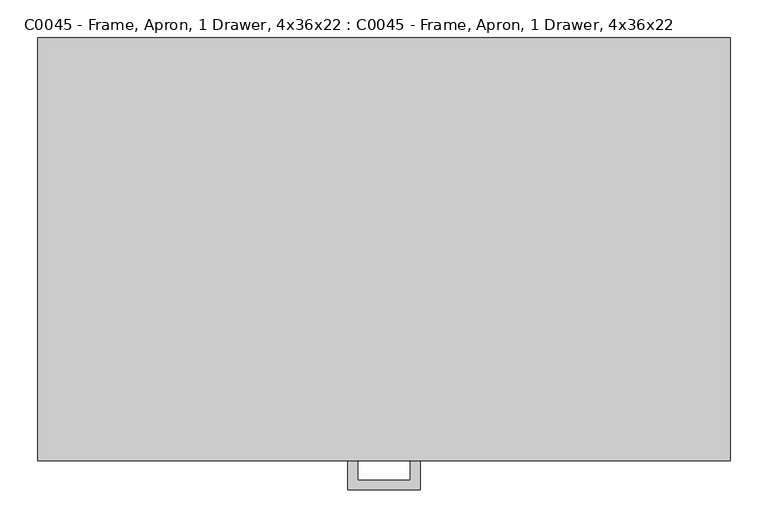
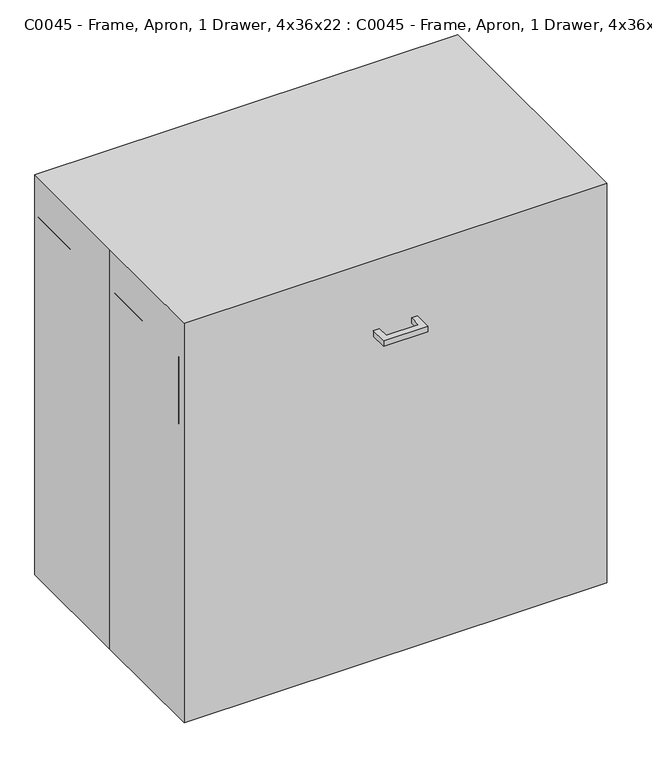
"""IFC4 building model written with IfcOpenShell, lengths in millimetres: proxy geometry, C0045 - Frame, Apron, 1 Drawer, 4x36x22 : C0045 - Frame, Apron, 1 Drawer, 4x36x22."""

import ifcopenshell
import ifcopenshell.guid

model = None  # the IFC model being written
_history = None  # IfcOwnerHistory: only IFC2X3 demands one
_inside = {}  # id of a spatial element -> (the spatial element, [elements in it])
_under = {}  # id of a project, library or spatial element -> (it, [spatial elements below it])
_declared = {}  # id of a project -> (the project, [libraries it declares])
_typed = {}  # id of a type object -> (the type object, [elements of that type])
_made_of = {}  # id of a material, layer set ... -> (it, [elements and type objects made of it])


def new_model(schema):
    """Start an empty IFC model of exactly this schema.

    Asked for "IFC4X3", IfcOpenShell would pick the latest addendum, in which some entities
    have other attributes; the version numbers below select the first issue.
    IFC2X3 requires an IfcOwnerHistory on every rooted entity: one is made here for all.
    """
    global model, _history
    if schema == "IFC4X3":
        model = ifcopenshell.file(schema_version=(4, 3, 0, 0))
    else:
        model = ifcopenshell.file(schema=schema)
    _inside.clear()
    _under.clear()
    _declared.clear()
    _typed.clear()
    _made_of.clear()
    _history = None
    if model.schema == "IFC2X3":
        org = make("IfcOrganization", Name="unknown")
        user = make(
            "IfcPersonAndOrganization",
            ThePerson=make("IfcPerson", FamilyName="unknown"),
            TheOrganization=org,
        )
        app = make(
            "IfcApplication",
            ApplicationDeveloper=org,
            Version="unknown",
            ApplicationFullName="unknown",
            ApplicationIdentifier="unknown",
        )
        _history = make(
            "IfcOwnerHistory",
            OwningUser=user,
            OwningApplication=app,
            ChangeAction="ADDED",
            CreationDate=0,
        )
    return model


def make(cls, **values):
    """One entity of the class cls with the attributes given. An attribute that is None is left unset."""
    return model.create_entity(
        cls, **{name: value for name, value in values.items() if value is not None}
    )


def rooted(cls, **values):
    """An entity with a GlobalId (a new one), such as an element, a storey or a relation."""
    return make(cls, GlobalId=ifcopenshell.guid.new(), OwnerHistory=_history, **values)


def si_unit(unit_type, name, prefix=None):
    """IfcSIUnit, for example si_unit("LENGTHUNIT", "METRE", prefix="MILLI")."""
    return make("IfcSIUnit", UnitType=unit_type, Prefix=prefix, Name=name)


def assignment(units):
    """IfcUnitAssignment: the units of a project."""
    return None if units is None else make("IfcUnitAssignment", Units=units)


def point(xyz):
    """IfcCartesianPoint."""
    return None if xyz is None else make("IfcCartesianPoint", Coordinates=xyz)


def direction(xyz):
    """IfcDirection."""
    return None if xyz is None else make("IfcDirection", DirectionRatios=xyz)


def frame(location, z_axis=None, x_axis=None):
    """IfcAxis2Placement3D, a coordinate frame: its origin and axes. An axis left out is left unset."""
    return make(
        "IfcAxis2Placement3D",
        Location=point(location),
        Axis=direction(z_axis),
        RefDirection=direction(x_axis),
    )


def origin():
    """The frame at (0, 0, 0) with its axes left unset."""
    return frame((0.0, 0.0, 0.0))


def origin_with_axes():
    """The frame at (0, 0, 0) with the z axis (0, 0, 1) and the x axis (1, 0, 0) written out."""
    return frame((0.0, 0.0, 0.0), z_axis=(0.0, 0.0, 1.0), x_axis=(1.0, 0.0, 0.0))


def place(relative_to, where):
    """IfcLocalPlacement: puts the frame where relative to a parent placement (None: the world)."""
    return make(
        "IfcLocalPlacement", PlacementRelTo=relative_to, RelativePlacement=where
    )


def context(
    kind, dimensions, precision=None, world=None, true_north=None, identifier=None
):
    """IfcGeometricRepresentationContext, for example the 3D "Model" context."""
    return make(
        "IfcGeometricRepresentationContext",
        ContextIdentifier=identifier,
        ContextType=kind,
        CoordinateSpaceDimension=dimensions,
        Precision=precision,
        WorldCoordinateSystem=world,
        TrueNorth=true_north,
    )


def project(units=None, contexts=None):
    """IfcProject with its units and contexts."""
    return rooted(
        "IfcProject",
        Name="project",
        RepresentationContexts=contexts,
        UnitsInContext=assignment(units),
    )


def spatial(cls, under=None, at=None, **own):
    """A site, building, storey or space (cls), placed at a placement, below another one or the project."""
    s = rooted(cls, ObjectPlacement=at, **own)
    if under is not None:
        _under.setdefault(under.id(), (under, []))[1].append(s)
    return s


def polyline(points):
    """IfcPolyline through the points."""
    return make("IfcPolyline", Points=[point(p) for p in points])


def outline(outer, holes=None, kind="AREA"):
    """IfcArbitraryClosedProfileDef: a profile drawn as a closed curve; with holes, ...WithVoids."""
    if holes is None:
        return make("IfcArbitraryClosedProfileDef", ProfileType=kind, OuterCurve=outer)
    return make(
        "IfcArbitraryProfileDefWithVoids",
        ProfileType=kind,
        OuterCurve=outer,
        InnerCurves=holes,
    )


def extrude(swept, where, along, depth):
    """IfcExtrudedAreaSolid: the profile swept, set in the frame where, extruded along a direction by depth."""
    return make(
        "IfcExtrudedAreaSolid",
        SweptArea=swept,
        Position=where,
        ExtrudedDirection=direction(along),
        Depth=depth,
    )


def shape(context_of_items, identifier, shape_type, items):
    """IfcShapeRepresentation: the items that make up one representation, for example the "Body"."""
    return make(
        "IfcShapeRepresentation",
        ContextOfItems=context_of_items,
        RepresentationIdentifier=identifier,
        RepresentationType=shape_type,
        Items=items,
    )


def source(mapping_origin, context_of_items, identifier, shape_type, items):
    """IfcRepresentationMap: a shape defined once, which mapped items show again and again."""
    return make(
        "IfcRepresentationMap",
        MappingOrigin=mapping_origin,
        MappedRepresentation=shape(context_of_items, identifier, shape_type, items),
    )


def transform(
    local_origin,
    x_axis=None,
    y_axis=None,
    z_axis=None,
    scale=None,
    scale2=None,
    scale3=None,
    uniform=True,
):
    """IfcCartesianTransformationOperator3D, or its non-uniform kind. x_axis, y_axis, z_axis: its Axis1, 2, 3."""
    if uniform:
        return make(
            "IfcCartesianTransformationOperator3D",
            Axis1=direction(x_axis),
            Axis2=direction(y_axis),
            LocalOrigin=point(local_origin),
            Scale=scale,
            Axis3=direction(z_axis),
        )
    return make(
        "IfcCartesianTransformationOperator3DnonUniform",
        Axis1=direction(x_axis),
        Axis2=direction(y_axis),
        LocalOrigin=point(local_origin),
        Scale=scale,
        Axis3=direction(z_axis),
        Scale2=scale2,
        Scale3=scale3,
    )


def mapped(mapping_source, mapping_target):
    """IfcMappedItem: shows the shape of a source again, moved by a transform."""
    return make(
        "IfcMappedItem", MappingSource=mapping_source, MappingTarget=mapping_target
    )


def made_of(thing, what):
    """Note that an element or type object is made of a material, layer set ...; save() writes the relation."""
    if what is not None:
        _made_of.setdefault(what.id(), (what, []))[1].append(thing)
    return thing


def element(
    cls,
    number,
    at=None,
    inside=None,
    cuts=None,
    type_object=None,
    material=None,
    context=None,
    identifier="Body",
    shape_type=None,
    held_by="IfcProductDefinitionShape",
    body=None,
    shapes=None,
    **own,
):
    """One element of the class cls, such as IfcWall. Its Tag is "e" and its number.

    at: its placement. inside: the storey or other place that contains it. cuts: it is an
    opening in that element (IfcRelVoidsElement). A single representation is given by context,
    identifier, shape_type and body (its items); several are given by shapes. held_by: the class
    of the entity that holds the representations. save() writes the other relations.
    """
    e = rooted(cls, Tag="e%d" % number, ObjectPlacement=at, **own)
    if body is not None:
        shapes = [shape(context, identifier, shape_type, body)]
    if shapes is not None:
        e.Representation = make(held_by, Representations=shapes)
    if inside is not None:
        _inside.setdefault(inside.id(), (inside, []))[1].append(e)
    if cuts is not None:
        rooted(
            "IfcRelVoidsElement", RelatingBuildingElement=cuts, RelatedOpeningElement=e
        )
    if type_object is not None:
        _typed.setdefault(type_object.id(), (type_object, []))[1].append(e)
    return made_of(e, material)


def aggregate(whole, parts):
    """IfcRelAggregates: a whole, such as a stair, and the parts it consists of."""
    return rooted("IfcRelAggregates", RelatingObject=whole, RelatedObjects=parts)


def save(model, path):
    """Write the relations noted so far, then the file.

    IfcRelAggregates (storeys below a building ...), IfcRelContainedInSpatialStructure (elements
    in a storey), IfcRelDefinesByType, IfcRelAssociatesMaterial and IfcRelDeclares: one each for
    every whole, place, type object, material and project.
    """
    for whole, parts in _under.values():
        aggregate(whole, parts)
    for where, things in _inside.values():
        rooted(
            "IfcRelContainedInSpatialStructure",
            RelatedElements=things,
            RelatingStructure=where,
        )
    for kind, things in _typed.values():
        rooted("IfcRelDefinesByType", RelatedObjects=things, RelatingType=kind)
    for what, things in _made_of.values():
        rooted("IfcRelAssociatesMaterial", RelatedObjects=things, RelatingMaterial=what)
    for by, libraries in _declared.values():
        rooted("IfcRelDeclares", RelatingContext=by, RelatedDefinitions=libraries)
    model.write(path)


def c0045_frame_apron_1_drawer_4x36x22_c0045_frame_apron_1_5ffb039a(model_context):
    return source(origin(), model_context, "Body", "SweptSolid", [
        extrude(outline(polyline([(-47.625, -317.5), (-47.625, -279.4), (-34.9409299, -279.4), (-34.9409299, -304.8159299), (34.9409299, -304.8159299), (34.9409299, -279.4), (47.625, -279.4), (47.625, -317.5), (-47.625, -317.5)])), frame((0.0, 0.0, 741.3462383), z_axis=(0.0, 0.0, 1.0), x_axis=(1.0, 0.0, 0.0)), (0.0, 0.0, 1.0), 12.7),
        extrude(outline(polyline([(-457.2, 279.4), (457.2, 279.4), (457.2, -279.4), (-457.2, -279.4), (-457.2, 0.0), (-457.2, 279.4)])), origin_with_axes(), (0.0, 0.0, 1.0), 914.4),
        extrude(outline(polyline([(438.15, -260.35), (438.15, 279.4), (457.2, 279.4), (457.2, -260.35), (438.15, -260.35)])), frame((0.0, 0.0, 673.0674767), z_axis=(0.0, 0.0, 1.0), x_axis=(1.0, 0.0, 0.0)), (0.0, 0.0, 1.0), 152.4),
        extrude(outline(polyline([(-457.2, -260.35), (-457.2, 279.4), (-438.15, 279.4), (-438.15, -260.35), (-457.2, -260.35)])), frame((0.0, 0.0, 673.0674767), z_axis=(0.0, 0.0, 1.0), x_axis=(1.0, 0.0, 0.0)), (0.0, 0.0, 1.0), 152.4),
        extrude(outline(polyline([(457.2, -279.4), (-457.2, -279.4), (-457.2, -260.35), (457.2, -260.35), (457.2, -279.4)])), frame((0.0, 0.0, 673.0674767), z_axis=(0.0, 0.0, 1.0), x_axis=(1.0, 0.0, 0.0)), (0.0, 0.0, 1.0), 152.4),
        extrude(outline(polyline([(438.15, 260.35), (438.15, -260.35), (-438.15, -260.35), (-438.15, 260.35), (438.15, 260.35)])), frame((0.0, 0.0, 673.0674767), z_axis=(0.0, 0.0, 1.0), x_axis=(1.0, 0.0, 0.0)), (0.0, 0.0, 1.0), 19.1166954),
        extrude(outline(polyline([(438.15, 260.35), (-438.15, 260.35), (-438.15, 279.4), (438.15, 279.4), (438.15, 260.35)])), frame((0.0, 0.0, 673.0674767), z_axis=(0.0, 0.0, 1.0), x_axis=(1.0, 0.0, 0.0)), (0.0, 0.0, 1.0), 133.35),
    ])


if __name__ == "__main__":
    model = new_model("IFC4")
    model_context = context("Model", 3, world=origin())
    ifc_project = project(units=[si_unit("LENGTHUNIT", "METRE", prefix="MILLI")], contexts=[model_context])
    site = spatial("IfcSite", under=ifc_project)
    building = spatial("IfcBuilding", under=site)
    placement = place(None, origin())
    c0045_frame_apron_1_drawer_4x36x22_c0045_frame_apron_1_shape = c0045_frame_apron_1_drawer_4x36x22_c0045_frame_apron_1_5ffb039a(model_context)
    element("IfcBuildingElementProxy", 1, Name="C0045 - Frame, Apron, 1 Drawer, 4x36x22 : C0045 - Frame, Apron, 1 Drawer, 4x36x22", ObjectType="C0045 - Frame, Apron, 1 Drawer, 4x36x22 : C0045 - Frame, Apron, 1 Drawer, 4x36x22", at=placement, inside=building, context=model_context, shape_type="MappedRepresentation", body=[
        mapped(c0045_frame_apron_1_drawer_4x36x22_c0045_frame_apron_1_shape, transform((0.0, 0.0, 0.0), x_axis=(1.0, 0.0, 0.0), y_axis=(0.0, 1.0, 0.0), z_axis=(0.0, 0.0, 1.0))),
    ])
    save(model, "model.ifc")

# Revit data of these elements
# Type "C0045 - Frame, Apron, 1 Drawer, 4x36x22 : C0045 - Frame, Apron, 1 Drawer, 4x36x22"
#   Watts2 = "0"
#   Watts1 = "0"
#   Unit_Issue = "EA"
#   UTIL_6_Misc = "-"
#   UTIL_5_NonMedGas = "-"
#   UTIL_4_MiscGas = "-"
#   UTIL_3_MedGas = "-"
#   UTIL_2_Elec = "-"
#   UTIL_1_WaterDrain = "-"
#   Nomenclature = "Frame, Apron, 1 Drawer, 4x36x22"
#   NSN = "6530"
#   Location [instance default] = ""
#   JSN = "C0045"
#   Fund_Source_VA = "-"
#   Fund_Source_Navy = "-"
#   Fund_Source_Army = "-"
#   Fund_Source_AF = "-"
#   ELEC_Volts2 = "0"
#   ELEC_Volts1 = "0"
#   ELEC_Phase2 = "0"
#   ELEC_Phase1 = "0"
#   ELEC_HertzSwitch = "0"
#   ELEC_HertzDependent = "0"
#   ELEC_Hertz = "0"
#   ELEC_Amps2 = "0"
#   ELEC_Amps1 = "0"
#   DetailDescription = "Apron frame with one standard drawer. Also referred to as a drawer frame or table frame. Used for a knee space as a combination frame and drawer to support a top between base cabinets or a base cabinet and a wall."
#   CAT_VA = "A"
#   CAT_Navy = "A"
#   CAT_IHS = "-"
#   CAT_Army = "A"
#   CAT_AF = "A"
#   BTUperhour = "0"
#   Weight_IP = 37
#   DIM_Width_IP = 3' - 0"
#   DIM_Height_IP = 3' - 0"
#   DIM_Depth_IP = 1' - 10"
#   Top Panel Material = none
#   Toe Panel Material = none
#   Side Panel Material = none
#   Shelf Panel Material = none
#   Drawer Front Material = none
#   Door Panel Material = none
#   Back Panel Material = none
#   Assembly Code = ""
# Element 1 (IfcBuildingElementProxy, "C0045 - Frame, Apron, 1 Drawer, 4x36x22 : C0045 - Frame, Apron, 1 Drawer, 4x36x22")
#   Materials on its faces: "Default metal", "EquipSpace"
# Materials
#   "Default metal": class "Unassigned", colour RGB 204 204 204, transparency 0
#   "EquipSpace": class "Unassigned", colour RGB 221 217 195, transparency 0.5
